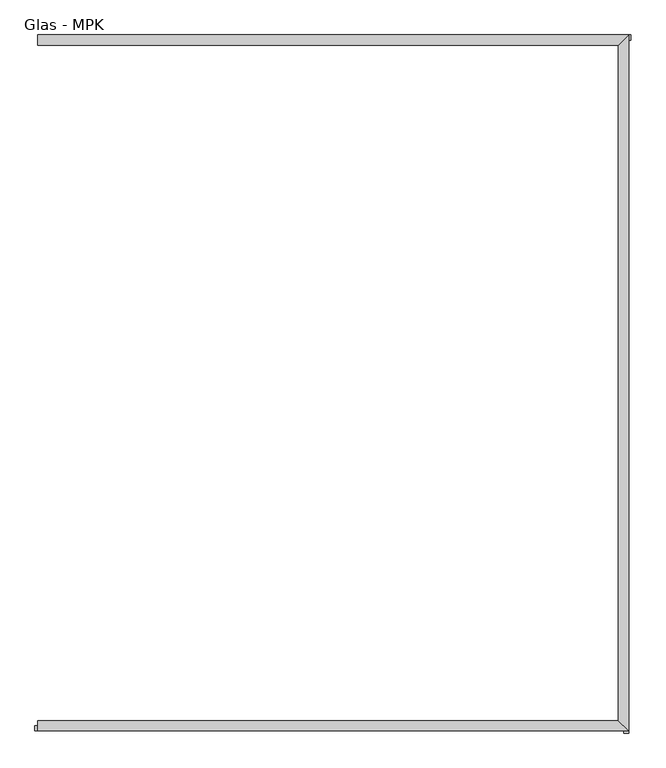
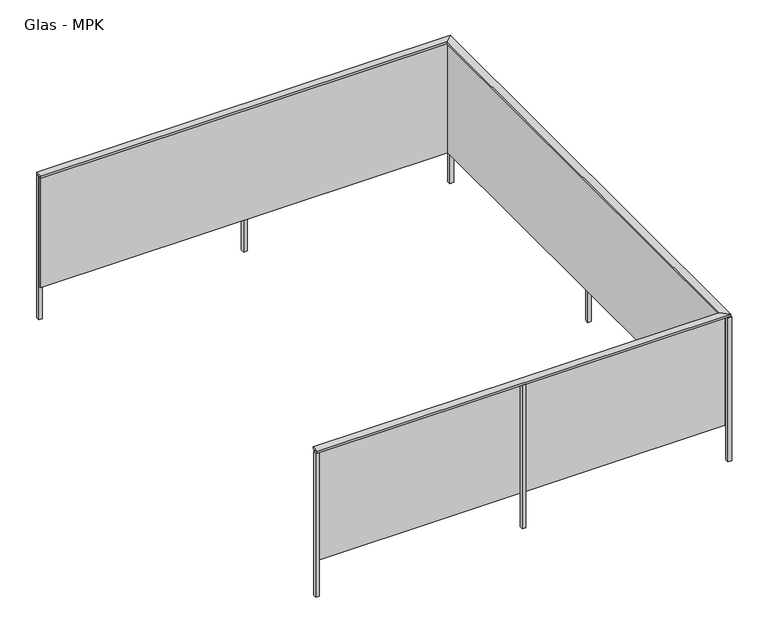
"""IFC4 building model written with IfcOpenShell, lengths in millimetres: railing geometry, Glas - MPK."""

from ifc_helpers import new_model, si_unit, frame, origin, place, context, project, spatial, polyline, outline, extrude, faceted_brep, source, transform, mapped, element, save


def glas_mpk_6e7e974a(model_context):
    return source(origin(), model_context, "Body", "SolidModel", [
        faceted_brep([(29194.1667192, -1196.642277, 9843.2628643), (29194.1667192, -1246.642277, 9843.2628643), (29194.1667192, -1246.642277, 9856.7371357), (29194.1667192, -1196.642277, 9856.7371357), (32034.1667192, -1196.642277, 9843.2628643), (31984.1667192, -1246.642277, 9843.2628643), (31984.1667192, -1246.642277, 9856.7371357), (32034.1667192, -1196.642277, 9856.7371357), (32034.1667192, -4537.3716232, 9843.2628643), (31984.1667192, -4487.3716232, 9843.2628643), (31984.1667192, -4487.3716232, 9856.7371357), (32034.1667192, -4537.3716232, 9856.7371357), (29194.1667192, -4537.3716232, 9843.2628643), (29194.1667192, -4537.3716232, 9856.7371357), (29194.1667192, -4487.3716232, 9856.7371357), (29194.1667192, -4487.3716232, 9843.2628643)], [[[0, 1, 2, 3]], [[1, 0, 4, 5]], [[2, 1, 5, 6]], [[3, 2, 6, 7]], [[0, 3, 7, 4]], [[5, 4, 8, 9]], [[6, 5, 9, 10]], [[7, 6, 10, 11]], [[4, 7, 11, 8]], [[12, 13, 14, 15]], [[9, 8, 12, 15]], [[10, 9, 15, 14]], [[11, 10, 14, 13]], [[8, 11, 13, 12]]]),
        faceted_brep([(29194.1667192, -1236.642277, 9842.8769824), (29194.1667192, -1222.4501531, 9842.8769824), (29194.1667192, -1222.4501531, 9042.8769824), (29194.1667192, -1236.642277, 9042.8769824), (31994.1667192, -1236.642277, 9842.8769824), (32008.3588432, -1222.4501531, 9842.8769824), (32008.3588432, -1222.4501531, 9042.8769824), (31994.1667192, -1236.642277, 9042.8769824), (31994.1667192, -4497.3716232, 9842.8769824), (32008.3588432, -4511.5637472, 9842.8769824), (32008.3588432, -4511.5637472, 9042.8769824), (31994.1667192, -4497.3716232, 9042.8769824), (29194.1667192, -4497.3716232, 9842.8769824), (29194.1667192, -4497.3716232, 9042.8769824), (29194.1667192, -4511.5637472, 9042.8769824), (29194.1667192, -4511.5637472, 9842.8769824)], [[[0, 1, 2, 3]], [[1, 0, 4, 5]], [[2, 1, 5, 6]], [[3, 2, 6, 7]], [[0, 3, 7, 4]], [[5, 4, 8, 9]], [[6, 5, 9, 10]], [[7, 6, 10, 11]], [[4, 7, 11, 8]], [[12, 13, 14, 15]], [[9, 8, 12, 15]], [[10, 9, 15, 14]], [[11, 10, 14, 13]], [[8, 11, 13, 12]]]),
        extrude(outline(polyline([(30625.4167192, -4512.3716232), (30625.4167192, -4537.3716232), (30600.4167192, -4537.3716232), (30600.4167192, -4512.3716232), (30625.4167192, -4512.3716232)])), frame((0.0, 0.0, 8800.0), z_axis=(0.0, 0.0, 1.0), x_axis=(1.0, 0.0, 0.0)), (0.0, 0.0, 1.0), 1043.2628643),
        extrude(outline(polyline([(32009.1667192, -2854.5069501), (32034.1667192, -2854.5069501), (32034.1667192, -2879.5069501), (32009.1667192, -2879.5069501), (32009.1667192, -2854.5069501)])), frame((0.0, 0.0, 8800.0), z_axis=(0.0, 0.0, 1.0), x_axis=(1.0, 0.0, 0.0)), (0.0, 0.0, 1.0), 1043.2628643),
        extrude(outline(polyline([(30600.4167192, -1221.642277), (30600.4167192, -1196.642277), (30625.4167192, -1196.642277), (30625.4167192, -1221.642277), (30600.4167192, -1221.642277)])), frame((0.0, 0.0, 8800.0), z_axis=(0.0, 0.0, 1.0), x_axis=(1.0, 0.0, 0.0)), (0.0, 0.0, 1.0), 1043.2628643),
        extrude(outline(polyline([(32009.1667192, -4522.3716232), (32034.1667192, -4522.3716232), (32034.1667192, -4547.3716232), (32009.1667192, -4547.3716232), (32009.1667192, -4522.3716232)])), frame((0.0, 0.0, 8800.0), z_axis=(0.0, 0.0, 1.0), x_axis=(1.0, 0.0, 0.0)), (0.0, 0.0, 1.0), 1043.2628643),
        extrude(outline(polyline([(32019.1667192, -1221.642277), (32019.1667192, -1196.642277), (32044.1667192, -1196.642277), (32044.1667192, -1221.642277), (32019.1667192, -1221.642277)])), frame((0.0, 0.0, 8800.0), z_axis=(0.0, 0.0, 1.0), x_axis=(1.0, 0.0, 0.0)), (0.0, 0.0, 1.0), 1043.2628643),
        extrude(outline(polyline([(29206.6667192, -4512.3716232), (29206.6667192, -4537.3716232), (29181.6667192, -4537.3716232), (29181.6667192, -4512.3716232), (29206.6667192, -4512.3716232)])), frame((0.0, 0.0, 8800.0), z_axis=(0.0, 0.0, 1.0), x_axis=(1.0, 0.0, 0.0)), (0.0, 0.0, 1.0), 1043.2628643),
        extrude(outline(polyline([(29194.1667192, -1221.642277), (29194.1667192, -1196.642277), (29219.1667192, -1196.642277), (29219.1667192, -1221.642277), (29194.1667192, -1221.642277)])), frame((0.0, 0.0, 8800.0), z_axis=(0.0, 0.0, 1.0), x_axis=(1.0, 0.0, 0.0)), (0.0, 0.0, 1.0), 1043.2628643),
    ])


if __name__ == "__main__":
    model = new_model("IFC4")
    model_context = context("Model", 3, world=origin())
    ifc_project = project(units=[si_unit("LENGTHUNIT", "METRE", prefix="MILLI")], contexts=[model_context])
    site = spatial("IfcSite", under=ifc_project)
    building = spatial("IfcBuilding", under=site)
    placement = place(None, origin())
    glas_mpk_shape = glas_mpk_6e7e974a(model_context)
    element("IfcRailing", 1, ObjectType="Glas - MPK", at=placement, inside=building, context=model_context, shape_type="MappedRepresentation", body=[
        mapped(glas_mpk_shape, transform((0.0, 0.0, 0.0), x_axis=(1.0, 0.0, 0.0), y_axis=(0.0, 1.0, 0.0), z_axis=(0.0, 0.0, 1.0))),
    ])
    save(model, "model.ifc")

# Revit data of these elements
# Element 1 (IfcRailing, "Glas - MPK")
#   Materials on its faces: "Metal - Aluminum", "Window - Glass"
# Materials
#   "Metal - Aluminum": class "Unassigned", colour RGB 247 247 247, transparency 0, Comments = "Rendering appearance not upgraded "
#   "Window - Glass": class "Glas", colour RGB 128 128 255, transparency 0.75
